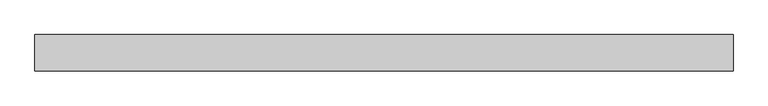
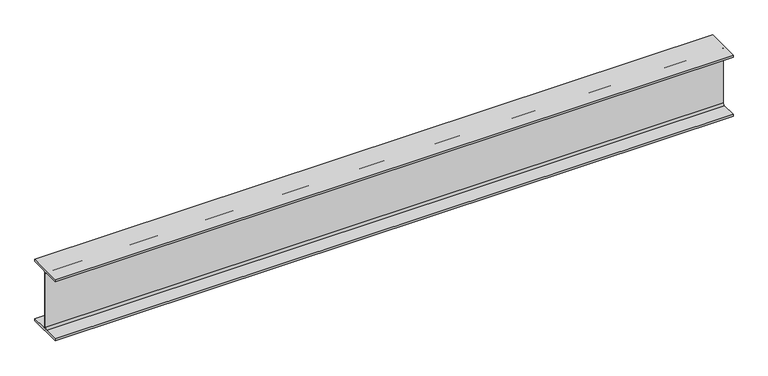
"""IFC4 building model written with IfcOpenShell, lengths in millimetres: beam geometry, Old_Steel Beam_H-KSD3502 : H_SB_ASB_H-200×200x8x12."""

from ifc_helpers import new_model, si_unit, point, frame, frame_2d, origin, place, context, project, spatial, polyline, circle_curve, trimmed, segment, composite_curve, outline, extrude, source, transform, mapped, element, save


def beam_382c5411(model_context):
    return source(origin(), model_context, "Body", "SweptSolid", [
        extrude(outline(composite_curve([segment(polyline([(82.5, -141.5), (82.5, -151.7), (-82.5, -151.7), (-82.5, -141.5), (-11.9, -141.5)]), True, "CONTINUOUS"), segment(trimmed(circle_curve(frame_2d((-11.9, -132.6)), 8.9), [point((-11.9, -141.5))], [point((-3.0, -132.6))], True, "CARTESIAN"), True, "CONTINUOUS"), segment(polyline([(-3.0, -132.6), (-3.0, 132.6)]), True, "CONTINUOUS"), segment(trimmed(circle_curve(frame_2d((-11.9, 132.6)), 8.9), [point((-3.0, 132.6))], [point((-11.9, 141.5))], True, "CARTESIAN"), True, "CONTINUOUS"), segment(polyline([(-11.9, 141.5), (-82.5, 141.5), (-82.5, 151.7), (82.5, 151.7), (82.5, 141.5), (11.9, 141.5)]), True, "CONTINUOUS"), segment(trimmed(circle_curve(frame_2d((11.9, 132.6)), 8.9), [point((11.9, 141.5))], [point((3.0, 132.6))], True, "CARTESIAN"), True, "CONTINUOUS"), segment(polyline([(3.0, 132.6), (3.0, -132.6)]), True, "CONTINUOUS"), segment(trimmed(circle_curve(frame_2d((11.9, -132.6)), 8.9), [point((3.0, -132.6))], [point((11.9, -141.5))], True, "CARTESIAN"), True, "CONTINUOUS"), segment(polyline([(11.9, -141.5), (82.5, -141.5)]), True, "CONTINUOUS")], self_intersect=False)), frame((-1449.1900782, 0.0, 0.0), z_axis=(1.0, 0.0, 0.0), x_axis=(0.0, 1.0, 0.0)), (0.0, 0.0, 1.0), 3170.9341584),
    ])


if __name__ == "__main__":
    model = new_model("IFC4")
    model_context = context("Model", 3, world=origin())
    ifc_project = project(units=[si_unit("LENGTHUNIT", "METRE", prefix="MILLI")], contexts=[model_context])
    site = spatial("IfcSite", under=ifc_project)
    building = spatial("IfcBuilding", under=site)
    placement = place(None, origin())
    beam_shape = beam_382c5411(model_context)
    element("IfcBeam", 1, ObjectType="Old_Steel Beam_H-KSD3502 : H_SB_ASB_H-200×200x8x12", at=placement, inside=building, context=model_context, shape_type="MappedRepresentation", body=[
        mapped(beam_shape, transform((0.0, 0.0, 0.0), x_axis=(1.0, 0.0, 0.0), y_axis=(0.0, 1.0, 0.0), z_axis=(0.0, 0.0, 1.0))),
    ])
    save(model, "model.ifc")

# Revit data of these elements
# Type "Old_Steel Beam_H-KSD3502 : H_SB_ASB_H-200×200x8x12"
#   Width = 20.0 cm
#   Web Thickness = 0.8 cm
#   Web Fillet = 1.3 cm
#   Warping Constant = 141376.0 cm⁶
#   Torsional Moment of Inertia = 26.2485 cm⁴
#   Torsional Modulus = 1.0 cm³
#   Section Area = 63.53 cm²
#   Plastic Modulus weak axis = 244.0 cm³
#   Plastic Modulus strong axis = 525.0 cm³
#   Perimeter = 1.16 m²/m
#   Nominal Weight = 49.90 kgf/m
#   Moment of Inertia weak axis = 1600.00 cm⁴
#   Moment of Inertia strong axis = 4720.00 cm⁴
#   Height = 20.0 cm
#   Flange Thickness = 1.2 cm
#   Elastic Modulus weak axis = 160.0 cm³
#   Elastic Modulus strong axis = 472.0 cm³
#   Centroid Vertical = 10.0 cm
#   Centroid Horizontal = 10.0 cm
#   Length [instance default] = 1.5240 m
#   Structural Material [instance default] = Steel, 45-345
#   Assembly Code = ""
# Element 1 (IfcBeam, "Old_Steel Beam_H-KSD3502 : H_SB_ASB_H-200×200x8x12")
#   Structural Material = none
# Materials
#   "Steel, 45-345": class "Metal", colour RGB 189 187 185, transparency 0, Description = "Steel 345 MPa", Cost = 0
